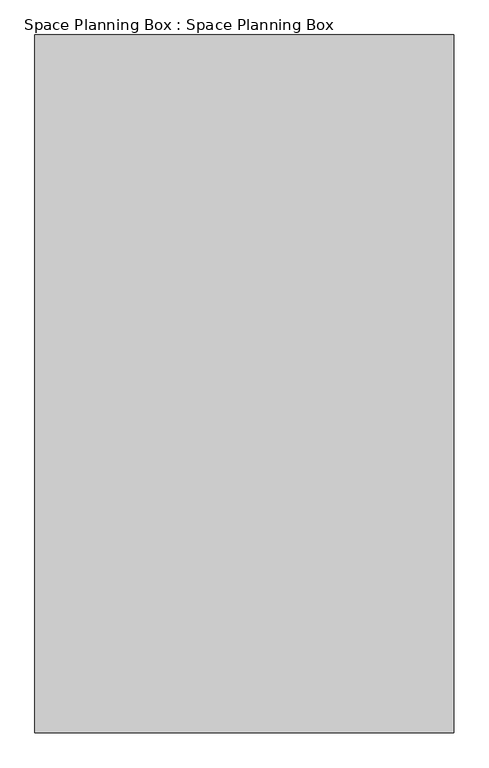
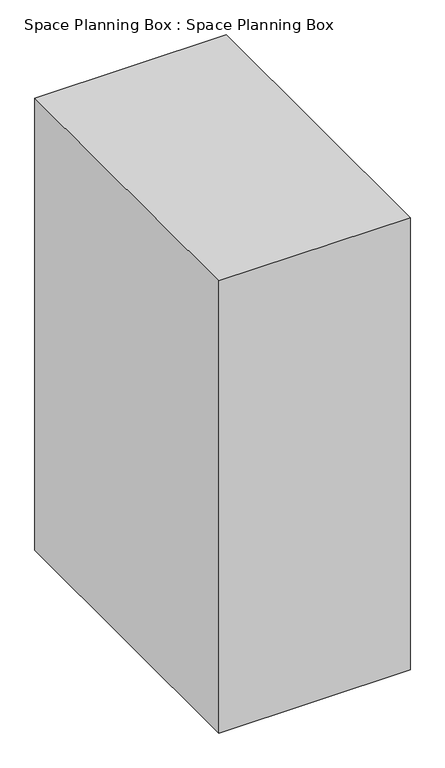
"""IFC4 building model written with IfcOpenShell, lengths in millimetres: proxy geometry, Space Planning Box : Space Planning Box."""

from ifc_helpers import new_model, si_unit, origin, origin_with_axes, place, context, project, spatial, polyline, outline, extrude, source, transform, mapped, element, save


def space_planning_box_space_planning_box_47b98be1(model_context):
    return source(origin(), model_context, "Body", "SweptSolid", [
        extrude(outline(polyline([(1200.0, 2000.0), (1200.0, -2000.0), (-1200.0, -2000.0), (-1200.0, 2000.0), (1200.0, 2000.0)])), origin_with_axes(), (0.0, 0.0, 1.0), 6000.0),
    ])


if __name__ == "__main__":
    model = new_model("IFC4")
    model_context = context("Model", 3, world=origin())
    ifc_project = project(units=[si_unit("LENGTHUNIT", "METRE", prefix="MILLI")], contexts=[model_context])
    site = spatial("IfcSite", under=ifc_project)
    building = spatial("IfcBuilding", under=site)
    placement = place(None, origin())
    space_planning_box_space_planning_box_shape = space_planning_box_space_planning_box_47b98be1(model_context)
    element("IfcBuildingElementProxy", 1, Name="Space Planning Box : Space Planning Box", ObjectType="Space Planning Box : Space Planning Box", at=placement, inside=building, context=model_context, shape_type="MappedRepresentation", body=[
        mapped(space_planning_box_space_planning_box_shape, transform((0.0, 0.0, 0.0), x_axis=(1.0, 0.0, 0.0), y_axis=(0.0, 1.0, 0.0), z_axis=(0.0, 0.0, 1.0))),
    ])
    save(model, "model.ifc")

# Revit data of these elements
# Type "Space Planning Box : Space Planning Box"
#   Type Comments = "..."
#   Room Name [instance default] = "?"
#   Assembly Code = "..."
#   Width [instance default] = 1524 mm
#   Program Area [instance default] = 0 m²
#   Length [instance default] = 1524 mm
#   Height [instance default] = 1524 mm
#   Area [instance default] = 2.32258 m²
#   Fill Color [instance default] = Cyan
#   Default Elevation = 0
# Element 1 (IfcBuildingElementProxy, "Space Planning Box : Space Planning Box")
#   Room Name = "Shower Room (F)"
#   Width = 2400 mm
#   Program Area = 31.5 m²
#   Length = 4000 mm
#   Height = 6000 mm
#   Area = 9.6 m²
#   Fill Color = Lavender
#   Materials on its faces: "Lavender"
# Materials
#   "Cyan": class "Generic", colour RGB 0 255 255, transparency 0.2, Cost = 0
#   "Lavender": class "Generic", colour RGB 186 85 211, transparency 0.2, Cost = 0
